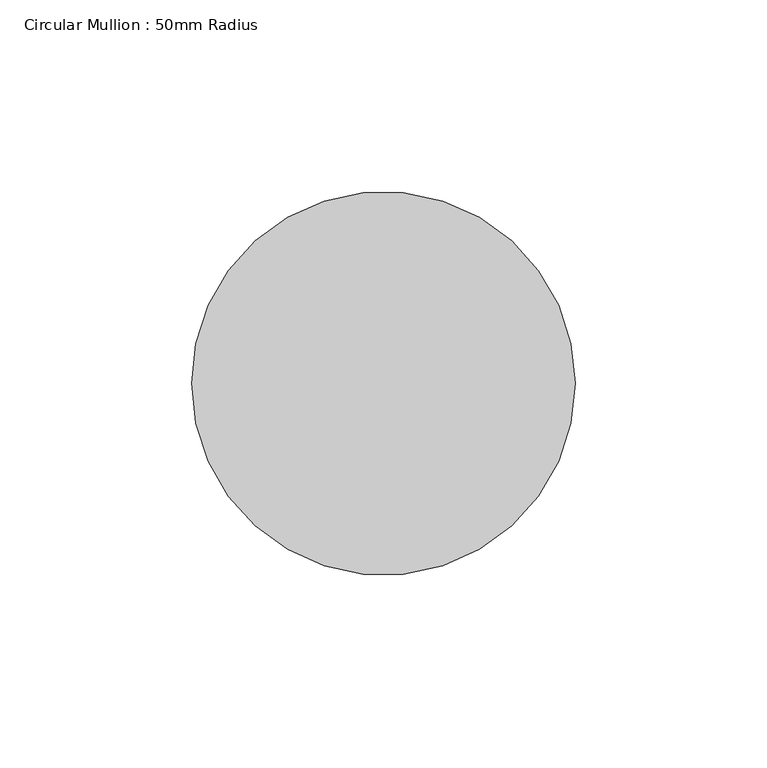
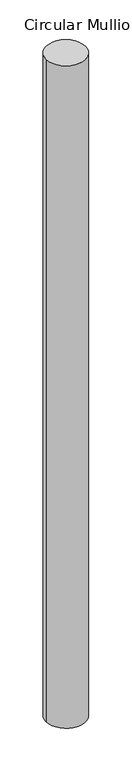
"""IFC4 building model written with IfcOpenShell, lengths in millimetres: member geometry, Circular Mullion : 50mm Radius."""

from ifc_helpers import new_model, si_unit, point, frame, origin, origin_2d, place, context, project, spatial, circle_curve, trimmed, segment, composite_curve, outline, extrude, source, transform, mapped, element, save


def circular_mullion_50mm_radius_982aae93(model_context):
    return source(origin(), model_context, "Body", "SweptSolid", [
        extrude(outline(composite_curve([segment(trimmed(circle_curve(origin_2d(), 50.0), [point((50.0, 0.0))], [point((-50.0, 0.0))], False, "CARTESIAN"), True, "CONTINUOUS"), segment(trimmed(circle_curve(origin_2d(), 50.0), [point((-50.0, 0.0))], [point((50.0, 0.0))], False, "CARTESIAN"), True, "CONTINUOUS")], self_intersect=False)), frame((0.0, 0.0, -1774.7382529), z_axis=(0.0, 0.0, 1.0), x_axis=(1.0, 0.0, 0.0)), (0.0, 0.0, 1.0), 1774.7382529),
    ])


if __name__ == "__main__":
    model = new_model("IFC4")
    model_context = context("Model", 3, world=origin())
    ifc_project = project(units=[si_unit("LENGTHUNIT", "METRE", prefix="MILLI")], contexts=[model_context])
    site = spatial("IfcSite", under=ifc_project)
    building = spatial("IfcBuilding", under=site)
    placement = place(None, origin())
    circular_mullion_50mm_radius_shape = circular_mullion_50mm_radius_982aae93(model_context)
    element("IfcMember", 1, ObjectType="Circular Mullion : 50mm Radius", at=placement, inside=building, context=model_context, shape_type="MappedRepresentation", body=[
        mapped(circular_mullion_50mm_radius_shape, transform((0.0, 0.0, 0.0), x_axis=(1.0, 0.0, 0.0), y_axis=(0.0, 1.0, 0.0), z_axis=(0.0, 0.0, 1.0))),
    ])
    save(model, "model.ifc")

# Revit data of these elements
# Type "Circular Mullion : 50mm Radius"
#   built-in parameter 1007350 = 0.164042 (stored number, unit not read)
# Element 1 (IfcMember, "Circular Mullion : 50mm Radius")
#   Materials on its faces: "Aluminium"
# Materials
#   "Aluminium": class "Metal", colour RGB 247 247 247, transparency 0, Description = "Aluminium 6061", Cost = 0
